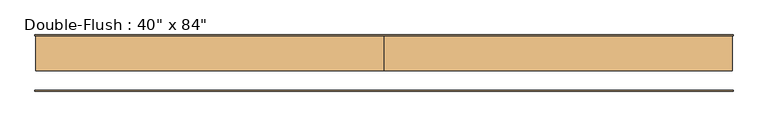
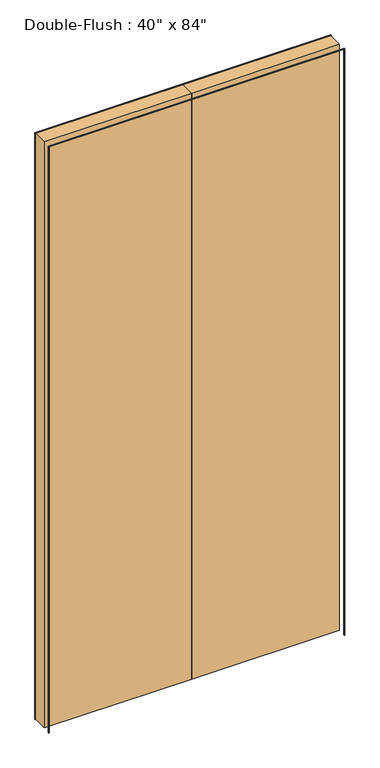
"""IFC4 building model written with IfcOpenShell, lengths in millimetres: door geometry."""

from ifc_helpers import new_model, si_unit, frame, origin, origin_with_axes, place, context, project, spatial, polyline, outline, extrude, source, transform, mapped, element, save


def door_839697f9(model_context):
    return source(origin(), model_context, "Body", "SweptSolid", [
        extrude(outline(polyline([(0.0, 39.6875), (508.0, 39.6875), (508.0, -11.1125), (0.0, -11.1125), (0.0, 39.6875)])), origin_with_axes(), (0.0, 0.0, 1.0), 2133.6),
        extrude(outline(polyline([(-508.0, 39.6875), (0.0, 39.6875), (0.0, -11.1125), (-508.0, -11.1125), (-508.0, 39.6875)])), origin_with_axes(), (0.0, 0.0, 1.0), 2133.6),
        extrude(outline(polyline([(2133.6, -508.0), (2133.6, 508.0), (0.0, 508.0), (0.0, 509.5875), (2135.1875, 509.5875), (2135.1875, -509.5875), (0.0, -509.5875), (0.0, -508.0), (2133.6, -508.0)])), frame((0.0, -41.275, 0.0), z_axis=(0.0, 1.0, 0.0), x_axis=(0.0, 0.0, 1.0)), (0.0, 0.0, 1.0), 1.5875),
        extrude(outline(polyline([(2133.6, -508.0), (2133.6, 508.0), (0.0, 508.0), (0.0, 509.5875), (2135.1875, 509.5875), (2135.1875, -509.5875), (0.0, -509.5875), (0.0, -508.0), (2133.6, -508.0)])), frame((0.0, 39.6875, 0.0), z_axis=(0.0, 1.0, 0.0), x_axis=(0.0, 0.0, 1.0)), (0.0, 0.0, 1.0), 1.5875),
    ])


if __name__ == "__main__":
    model = new_model("IFC4")
    model_context = context("Model", 3, world=origin())
    ifc_project = project(units=[si_unit("LENGTHUNIT", "METRE", prefix="MILLI")], contexts=[model_context])
    site = spatial("IfcSite", under=ifc_project)
    building = spatial("IfcBuilding", under=site)
    placement = place(None, origin())
    door_shape = door_839697f9(model_context)
    element("IfcDoor", 1, ObjectType="Double-Flush : 40\" x 84\"", at=placement, inside=building, context=model_context, shape_type="MappedRepresentation", body=[
        mapped(door_shape, transform((0.0, 0.0, 0.0), x_axis=(1.0, 0.0, 0.0), y_axis=(0.0, 1.0, 0.0), z_axis=(0.0, 0.0, 1.0))),
    ])
    save(model, "model.ifc")

# Revit data of these elements
# Type "Double-Flush : 40\" x 84\""
#   Type Mark = "41"
#   Assembly Code = "C1020"
#   Thickness = 0' - 2"
#   Height = 7' - 0"
#   Trim Projection Ext = 0' - 0 1/16"
#   Trim Projection Int = 0' - 0 1/16"
#   Trim Width = 0' - 0 1/16"
#   Width = 3' - 4"
#   Door Material = Door - Panel
#   Frame Material = Door - Frame
#   Function = (empty or 0)
#   Wall Closure = (empty or 0)
# Element 1 (IfcDoor, "Double-Flush : 40\" x 84\"")
#   Materials on its faces: "Door - Frame", "Door - Panel"
# Materials
#   "Door - Panel": class "Wood", colour RGB 210 159 95, transparency 0
#   "Door - Frame": class "Miscellaneous", colour RGB 118 70 51, transparency 0
